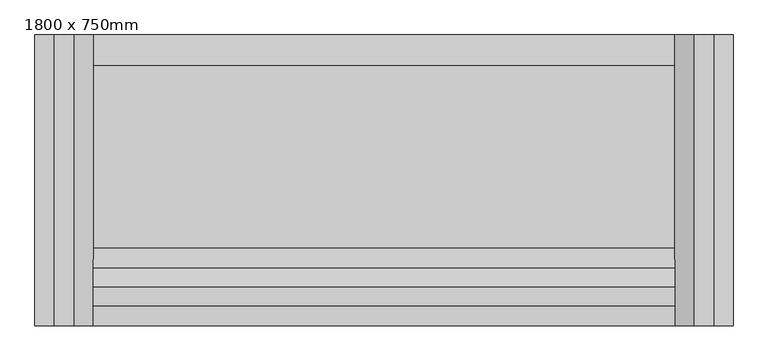
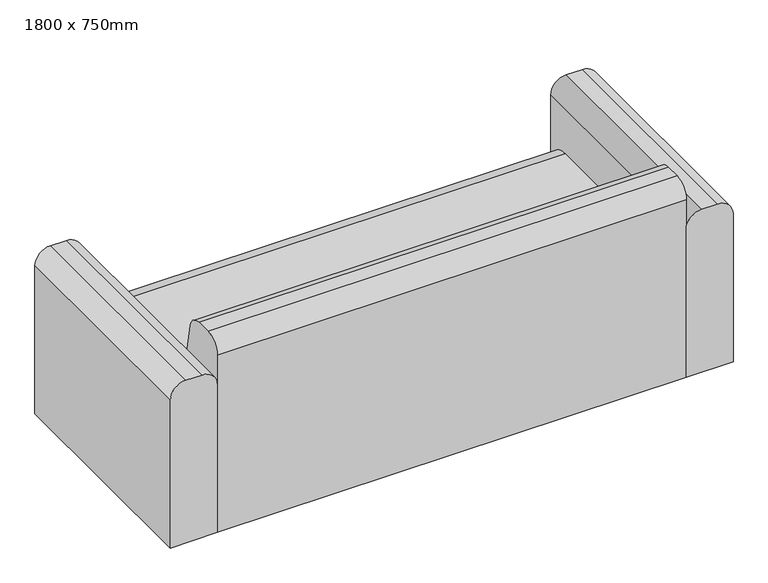
"""IFC4 building model written with IfcOpenShell, lengths in millimetres: furniture geometry, ソファ－I型 : 1800 x 750mm."""

from ifc_helpers import new_model, si_unit, point, frame, frame_2d, origin, place, context, project, spatial, polyline, circle_curve, trimmed, segment, composite_curve, outline, extrude, source, transform, mapped, element, save


def furniture_1800_x_750mm_5b3da114(model_context):
    return source(origin(), model_context, "Body", "SweptSolid", [
        extrude(outline(composite_curve([segment(trimmed(circle_curve(frame_2d((500.0, -850.0)), 50.0), [point((550.0, -850.0))], [point((500.0, -900.0))], False, "CARTESIAN"), True, "CONTINUOUS"), segment(polyline([(500.0, -900.0), (0.0, -900.0), (0.0, -750.0), (500.0, -750.0)]), True, "CONTINUOUS"), segment(trimmed(circle_curve(frame_2d((500.0, -800.0)), 50.0), [point((500.0, -750.0))], [point((550.0, -800.0))], False, "CARTESIAN"), True, "CONTINUOUS"), segment(polyline([(550.0, -800.0), (550.0, -850.0)]), True, "CONTINUOUS")], self_intersect=False)), frame((0.0, -375.0, 0.0), z_axis=(0.0, 1.0, 0.0), x_axis=(0.0, 0.0, 1.0)), (0.0, 0.0, 1.0), 750.0),
        extrude(outline(composite_curve([segment(polyline([(550.0, 850.0), (550.0, 800.0)]), True, "CONTINUOUS"), segment(trimmed(circle_curve(frame_2d((500.0, 800.0)), 50.0), [point((550.0, 800.0))], [point((500.0, 750.0))], False, "CARTESIAN"), True, "CONTINUOUS"), segment(polyline([(500.0, 750.0), (0.0, 750.0), (0.0, 900.0), (500.0, 900.0)]), True, "CONTINUOUS"), segment(trimmed(circle_curve(frame_2d((500.0, 850.0)), 50.0), [point((500.0, 900.0))], [point((550.0, 850.0))], False, "CARTESIAN"), True, "CONTINUOUS")], self_intersect=False)), frame((0.0, -375.0, 0.0), z_axis=(0.0, 1.0, 0.0), x_axis=(0.0, 0.0, 1.0)), (0.0, 0.0, 1.0), 750.0),
        extrude(outline(composite_curve([segment(polyline([(-226.9611614, 609.8058068), (-175.0, 350.0), (295.0, 350.0)]), True, "CONTINUOUS"), segment(trimmed(circle_curve(frame_2d((295.0, 270.0)), 80.0), [point((295.0, 350.0))], [point((375.0, 270.0))], False, "CARTESIAN"), True, "CONTINUOUS"), segment(polyline([(375.0, 270.0), (375.0, 60.0), (305.0, 60.0), (305.0, 0.0), (-375.0, 0.0), (-375.0, 600.0)]), True, "CONTINUOUS"), segment(trimmed(circle_curve(frame_2d((-325.0, 600.0)), 50.0), [point((-375.0, 600.0))], [point((-325.0, 650.0))], False, "CARTESIAN"), True, "CONTINUOUS"), segment(polyline([(-325.0, 650.0), (-275.9901951, 650.0)]), True, "CONTINUOUS"), segment(trimmed(circle_curve(frame_2d((-275.9901951, 600.0)), 50.0), [point((-275.9901951, 650.0))], [point((-226.9611614, 609.8058068))], False, "CARTESIAN"), True, "CONTINUOUS")], self_intersect=False)), frame((-750.0, 0.0, 0.0), z_axis=(1.0, 0.0, 0.0), x_axis=(0.0, 1.0, 0.0)), (0.0, 0.0, 1.0), 1500.0),
    ])


if __name__ == "__main__":
    model = new_model("IFC4")
    model_context = context("Model", 3, world=origin())
    ifc_project = project(units=[si_unit("LENGTHUNIT", "METRE", prefix="MILLI")], contexts=[model_context])
    site = spatial("IfcSite", under=ifc_project)
    building = spatial("IfcBuilding", under=site)
    placement = place(None, origin())
    furniture_1800_x_750mm_shape = furniture_1800_x_750mm_5b3da114(model_context)
    element("IfcFurniture", 1, ObjectType="ソファ－I型 : 1800 x 750mm", at=placement, inside=building, context=model_context, shape_type="MappedRepresentation", body=[
        mapped(furniture_1800_x_750mm_shape, transform((0.0, 0.0, 0.0), x_axis=(1.0, 0.0, 0.0), y_axis=(0.0, 1.0, 0.0), z_axis=(0.0, 0.0, 1.0))),
    ])
    save(model, "model.ifc")

# Revit data of these elements
# Project information
#   プロジェクト発行日 = "発行日"
#   プロジェクト ステータス = "プロジェクト ステータス"
#   クライアント名 = "オーナ"
#   計画地住所 = "ここにアドレスを入力"
#   プロジェクト名 = "プロジェクト名"
#   プロジェクト番号 = "0001"
# Type "ソファ－I型 : 1800 x 750mm"
#   Keynote = "12490.Y1"
#   座面高さ = 350 mm
#   幅 = 1800 mm
#   奥行き = 750 mm
#   本体 = モチアミ - 無地 - グレー
#   Default Elevation = 0
# Element 1 (IfcFurniture, "ソファ－I型 : 1800 x 750mm")
#   Materials on its faces: "モチアミ - 無地 - グレー"
# Materials
#   "モチアミ - 無地 - グレー": class "モチアミ", colour RGB 65 63 65, transparency 0, Cost = 0
